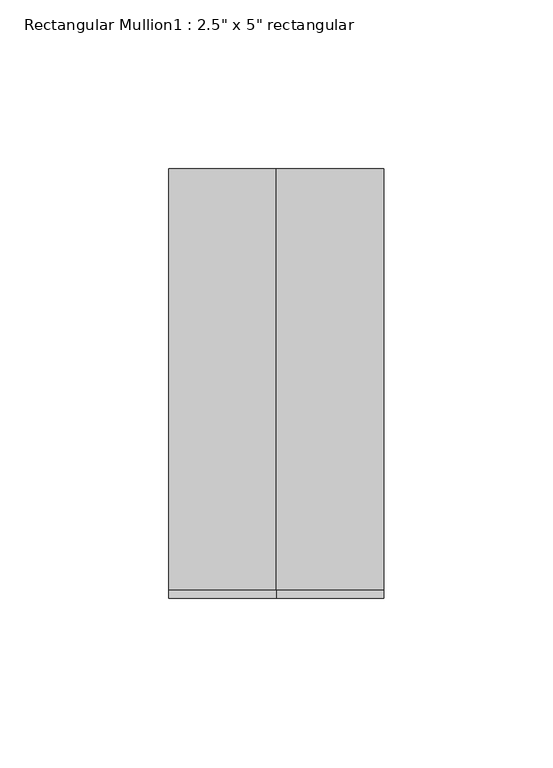
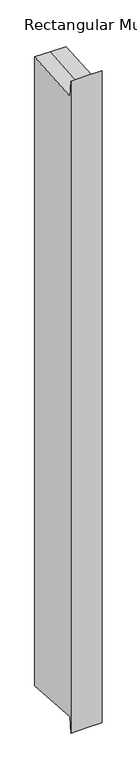
"""IFC4 building model written with IfcOpenShell, lengths in millimetres: member geometry."""

import ifcopenshell
import ifcopenshell.guid

model = None  # the IFC model being written
_history = None  # IfcOwnerHistory: only IFC2X3 demands one
_inside = {}  # id of a spatial element -> (the spatial element, [elements in it])
_under = {}  # id of a project, library or spatial element -> (it, [spatial elements below it])
_declared = {}  # id of a project -> (the project, [libraries it declares])
_typed = {}  # id of a type object -> (the type object, [elements of that type])
_made_of = {}  # id of a material, layer set ... -> (it, [elements and type objects made of it])


def new_model(schema):
    """Start an empty IFC model of exactly this schema.

    Asked for "IFC4X3", IfcOpenShell would pick the latest addendum, in which some entities
    have other attributes; the version numbers below select the first issue.
    IFC2X3 requires an IfcOwnerHistory on every rooted entity: one is made here for all.
    """
    global model, _history
    if schema == "IFC4X3":
        model = ifcopenshell.file(schema_version=(4, 3, 0, 0))
    else:
        model = ifcopenshell.file(schema=schema)
    _inside.clear()
    _under.clear()
    _declared.clear()
    _typed.clear()
    _made_of.clear()
    _history = None
    if model.schema == "IFC2X3":
        org = make("IfcOrganization", Name="unknown")
        user = make(
            "IfcPersonAndOrganization",
            ThePerson=make("IfcPerson", FamilyName="unknown"),
            TheOrganization=org,
        )
        app = make(
            "IfcApplication",
            ApplicationDeveloper=org,
            Version="unknown",
            ApplicationFullName="unknown",
            ApplicationIdentifier="unknown",
        )
        _history = make(
            "IfcOwnerHistory",
            OwningUser=user,
            OwningApplication=app,
            ChangeAction="ADDED",
            CreationDate=0,
        )
    return model


def make(cls, **values):
    """One entity of the class cls with the attributes given. An attribute that is None is left unset."""
    return model.create_entity(
        cls, **{name: value for name, value in values.items() if value is not None}
    )


def rooted(cls, **values):
    """An entity with a GlobalId (a new one), such as an element, a storey or a relation."""
    return make(cls, GlobalId=ifcopenshell.guid.new(), OwnerHistory=_history, **values)


def si_unit(unit_type, name, prefix=None):
    """IfcSIUnit, for example si_unit("LENGTHUNIT", "METRE", prefix="MILLI")."""
    return make("IfcSIUnit", UnitType=unit_type, Prefix=prefix, Name=name)


def assignment(units):
    """IfcUnitAssignment: the units of a project."""
    return None if units is None else make("IfcUnitAssignment", Units=units)


def point(xyz):
    """IfcCartesianPoint."""
    return None if xyz is None else make("IfcCartesianPoint", Coordinates=xyz)


def direction(xyz):
    """IfcDirection."""
    return None if xyz is None else make("IfcDirection", DirectionRatios=xyz)


def frame(location, z_axis=None, x_axis=None):
    """IfcAxis2Placement3D, a coordinate frame: its origin and axes. An axis left out is left unset."""
    return make(
        "IfcAxis2Placement3D",
        Location=point(location),
        Axis=direction(z_axis),
        RefDirection=direction(x_axis),
    )


def origin():
    """The frame at (0, 0, 0) with its axes left unset."""
    return frame((0.0, 0.0, 0.0))


def place(relative_to, where):
    """IfcLocalPlacement: puts the frame where relative to a parent placement (None: the world)."""
    return make(
        "IfcLocalPlacement", PlacementRelTo=relative_to, RelativePlacement=where
    )


def context(
    kind, dimensions, precision=None, world=None, true_north=None, identifier=None
):
    """IfcGeometricRepresentationContext, for example the 3D "Model" context."""
    return make(
        "IfcGeometricRepresentationContext",
        ContextIdentifier=identifier,
        ContextType=kind,
        CoordinateSpaceDimension=dimensions,
        Precision=precision,
        WorldCoordinateSystem=world,
        TrueNorth=true_north,
    )


def project(units=None, contexts=None):
    """IfcProject with its units and contexts."""
    return rooted(
        "IfcProject",
        Name="project",
        RepresentationContexts=contexts,
        UnitsInContext=assignment(units),
    )


def spatial(cls, under=None, at=None, **own):
    """A site, building, storey or space (cls), placed at a placement, below another one or the project."""
    s = rooted(cls, ObjectPlacement=at, **own)
    if under is not None:
        _under.setdefault(under.id(), (under, []))[1].append(s)
    return s


def faces_of(points, faces, orient=None, outer=None):
    """IfcFace entities. A face is a list of loops; a loop is a list of indices into points, from 0.

    orient and outer hold one flag for each loop. By default every Orientation is true, the
    first loop of a face is its IfcFaceOuterBound and the others are IfcFaceBound.
    """
    made = []
    for i, loops in enumerate(faces):
        bounds = []
        for j, loop in enumerate(loops):
            is_outer = j == 0 if outer is None else outer[i][j]
            bounds.append(
                make(
                    "IfcFaceOuterBound" if is_outer else "IfcFaceBound",
                    Bound=make("IfcPolyLoop", Polygon=[points[k] for k in loop]),
                    Orientation=True if orient is None else orient[i][j],
                )
            )
        made.append(make("IfcFace", Bounds=bounds))
    return made


def faceted_brep(points, faces, orient=None, outer=None, voids=None):
    """IfcFacetedBrep: a solid bounded by flat faces; with voids (closed shells), ...WithVoids."""
    shared = [point(p) for p in points]
    hull = make("IfcClosedShell", CfsFaces=faces_of(shared, faces, orient, outer))
    if voids is None:
        return make("IfcFacetedBrep", Outer=hull)
    return make(
        "IfcFacetedBrepWithVoids",
        Outer=hull,
        Voids=[
            make(cls, CfsFaces=faces_of(shared, fs, o, b)) for cls, fs, o, b in voids
        ],
    )


def shape(context_of_items, identifier, shape_type, items):
    """IfcShapeRepresentation: the items that make up one representation, for example the "Body"."""
    return make(
        "IfcShapeRepresentation",
        ContextOfItems=context_of_items,
        RepresentationIdentifier=identifier,
        RepresentationType=shape_type,
        Items=items,
    )


def source(mapping_origin, context_of_items, identifier, shape_type, items):
    """IfcRepresentationMap: a shape defined once, which mapped items show again and again."""
    return make(
        "IfcRepresentationMap",
        MappingOrigin=mapping_origin,
        MappedRepresentation=shape(context_of_items, identifier, shape_type, items),
    )


def transform(
    local_origin,
    x_axis=None,
    y_axis=None,
    z_axis=None,
    scale=None,
    scale2=None,
    scale3=None,
    uniform=True,
):
    """IfcCartesianTransformationOperator3D, or its non-uniform kind. x_axis, y_axis, z_axis: its Axis1, 2, 3."""
    if uniform:
        return make(
            "IfcCartesianTransformationOperator3D",
            Axis1=direction(x_axis),
            Axis2=direction(y_axis),
            LocalOrigin=point(local_origin),
            Scale=scale,
            Axis3=direction(z_axis),
        )
    return make(
        "IfcCartesianTransformationOperator3DnonUniform",
        Axis1=direction(x_axis),
        Axis2=direction(y_axis),
        LocalOrigin=point(local_origin),
        Scale=scale,
        Axis3=direction(z_axis),
        Scale2=scale2,
        Scale3=scale3,
    )


def mapped(mapping_source, mapping_target):
    """IfcMappedItem: shows the shape of a source again, moved by a transform."""
    return make(
        "IfcMappedItem", MappingSource=mapping_source, MappingTarget=mapping_target
    )


def made_of(thing, what):
    """Note that an element or type object is made of a material, layer set ...; save() writes the relation."""
    if what is not None:
        _made_of.setdefault(what.id(), (what, []))[1].append(thing)
    return thing


def element(
    cls,
    number,
    at=None,
    inside=None,
    cuts=None,
    type_object=None,
    material=None,
    context=None,
    identifier="Body",
    shape_type=None,
    held_by="IfcProductDefinitionShape",
    body=None,
    shapes=None,
    **own,
):
    """One element of the class cls, such as IfcWall. Its Tag is "e" and its number.

    at: its placement. inside: the storey or other place that contains it. cuts: it is an
    opening in that element (IfcRelVoidsElement). A single representation is given by context,
    identifier, shape_type and body (its items); several are given by shapes. held_by: the class
    of the entity that holds the representations. save() writes the other relations.
    """
    e = rooted(cls, Tag="e%d" % number, ObjectPlacement=at, **own)
    if body is not None:
        shapes = [shape(context, identifier, shape_type, body)]
    if shapes is not None:
        e.Representation = make(held_by, Representations=shapes)
    if inside is not None:
        _inside.setdefault(inside.id(), (inside, []))[1].append(e)
    if cuts is not None:
        rooted(
            "IfcRelVoidsElement", RelatingBuildingElement=cuts, RelatedOpeningElement=e
        )
    if type_object is not None:
        _typed.setdefault(type_object.id(), (type_object, []))[1].append(e)
    return made_of(e, material)


def aggregate(whole, parts):
    """IfcRelAggregates: a whole, such as a stair, and the parts it consists of."""
    return rooted("IfcRelAggregates", RelatingObject=whole, RelatedObjects=parts)


def save(model, path):
    """Write the relations noted so far, then the file.

    IfcRelAggregates (storeys below a building ...), IfcRelContainedInSpatialStructure (elements
    in a storey), IfcRelDefinesByType, IfcRelAssociatesMaterial and IfcRelDeclares: one each for
    every whole, place, type object, material and project.
    """
    for whole, parts in _under.values():
        aggregate(whole, parts)
    for where, things in _inside.values():
        rooted(
            "IfcRelContainedInSpatialStructure",
            RelatedElements=things,
            RelatingStructure=where,
        )
    for kind, things in _typed.values():
        rooted("IfcRelDefinesByType", RelatedObjects=things, RelatingType=kind)
    for what, things in _made_of.values():
        rooted("IfcRelAssociatesMaterial", RelatedObjects=things, RelatingMaterial=what)
    for by, libraries in _declared.values():
        rooted("IfcRelDeclares", RelatingContext=by, RelatedDefinitions=libraries)
    model.write(path)


def member_995572cb(model_context):
    return source(origin(), model_context, "Body", "Brep", [
        faceted_brep([(-31.75, 63.5, 4.5282284), (0.0, 63.5, 4.5282284), (31.75, 63.5, 4.5282284), (31.75, 63.5, -1343.9489353), (0.0, 63.5, -1343.9489353), (-31.75, 63.5, -1343.9489353), (-31.75, -63.5, 29.4471051), (-31.75, -61.0333155, -4.5163328), (-31.75, -61.0333155, -1334.904374), (-31.75, -63.5, -1368.8678119), (31.75, -63.5, 29.4471051), (0.0, -63.5, 29.4471051), (0.0, -63.5, -1368.8678119), (31.75, -63.5, -1368.8678119), (31.75, -61.0333155, -4.5163328), (31.75, -61.0333155, -1334.904374), (0.0, -61.0333155, -4.5163328), (0.0, -61.0333155, -1334.904374)], [[[0, 1, 2, 3, 4, 5]], [[6, 7, 0, 5, 8, 9]], [[10, 11, 6, 9, 12, 13]], [[2, 14, 10, 13, 15, 3]], [[2, 1, 16, 14]], [[1, 0, 7, 16]], [[7, 6, 11, 16]], [[11, 10, 14, 16]], [[3, 15, 17, 4]], [[15, 13, 12, 17]], [[12, 9, 8, 17]], [[8, 5, 4, 17]]]),
    ])


if __name__ == "__main__":
    model = new_model("IFC4")
    model_context = context("Model", 3, world=origin())
    ifc_project = project(units=[si_unit("LENGTHUNIT", "METRE", prefix="MILLI")], contexts=[model_context])
    site = spatial("IfcSite", under=ifc_project)
    building = spatial("IfcBuilding", under=site)
    placement = place(None, origin())
    member_shape = member_995572cb(model_context)
    element("IfcMember", 1, ObjectType="Rectangular Mullion1 : 2.5\" x 5\" rectangular", at=placement, inside=building, context=model_context, shape_type="MappedRepresentation", body=[
        mapped(member_shape, transform((0.0, 0.0, 0.0), x_axis=(1.0, 0.0, 0.0), y_axis=(0.0, 1.0, 0.0), z_axis=(0.0, 0.0, 1.0))),
    ])
    save(model, "model.ifc")

# Revit data of these elements
# Type "Rectangular Mullion1 : 2.5\" x 5\" rectangular"
#   built-in parameter 1007304 = 0.416667 (stored number, unit not read)
#   built-in parameter 1007301 = 0.104167 (stored number, unit not read)
#   built-in parameter 1007300 = 0.104167 (stored number, unit not read)
# Element 1 (IfcMember, "Rectangular Mullion1 : 2.5\" x 5\" rectangular")
#   Materials on its faces: "support-frame"
# Materials
#   "support-frame": class "Unassigned", colour RGB 233 233 233, transparency 0, Cost = 0
